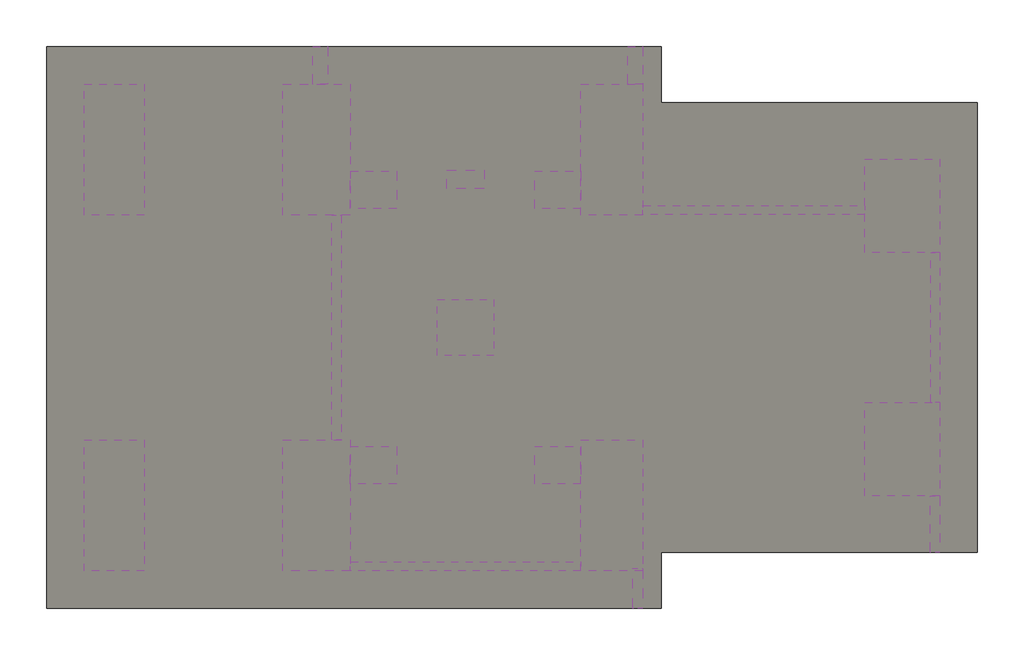
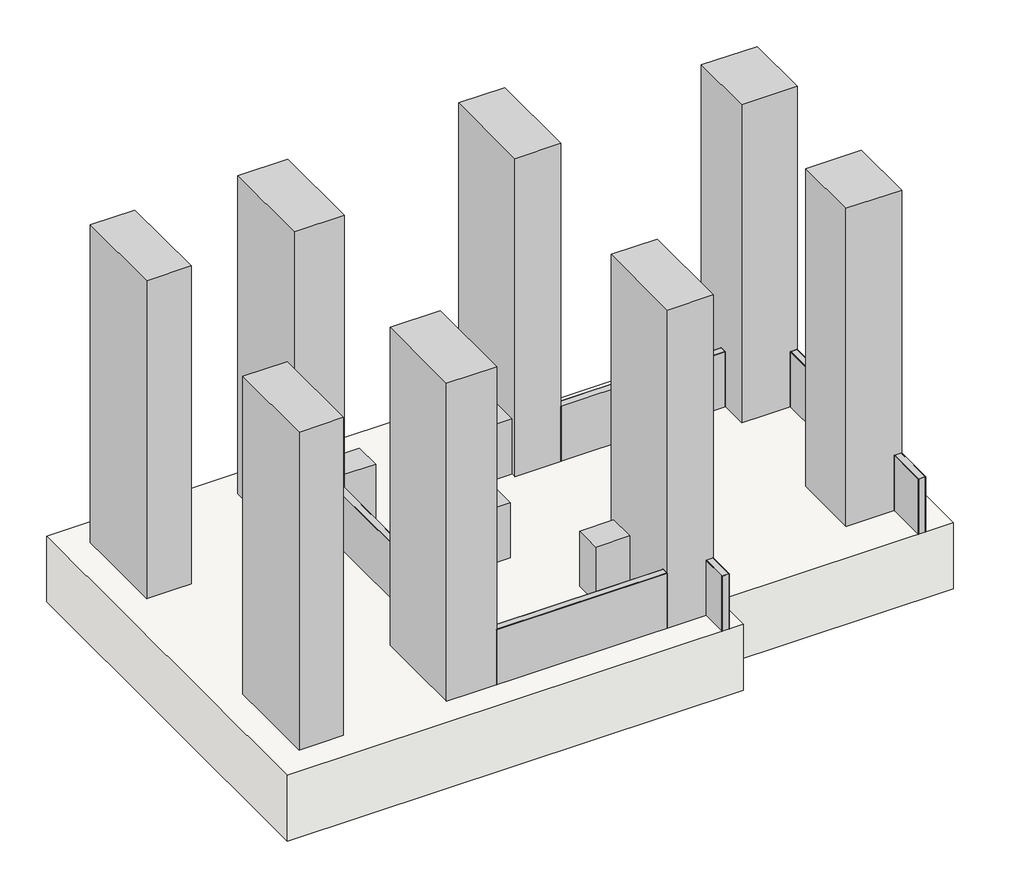
# One storey: 14 columns, 8 beams, 1 slab.
"""IFC4 building model written with IfcOpenShell, lengths in millimetres."""

import ifcopenshell
import ifcopenshell.guid

model = None  # the IFC model being written
_history = None  # IfcOwnerHistory: only IFC2X3 demands one
_inside = {}  # id of a spatial element -> (the spatial element, [elements in it])
_under = {}  # id of a project, library or spatial element -> (it, [spatial elements below it])
_declared = {}  # id of a project -> (the project, [libraries it declares])
_typed = {}  # id of a type object -> (the type object, [elements of that type])
_made_of = {}  # id of a material, layer set ... -> (it, [elements and type objects made of it])


def new_model(schema):
    """Start an empty IFC model of exactly this schema.

    Asked for "IFC4X3", IfcOpenShell would pick the latest addendum, in which some entities
    have other attributes; the version numbers below select the first issue.
    IFC2X3 requires an IfcOwnerHistory on every rooted entity: one is made here for all.
    """
    global model, _history
    if schema == "IFC4X3":
        model = ifcopenshell.file(schema_version=(4, 3, 0, 0))
    else:
        model = ifcopenshell.file(schema=schema)
    _inside.clear()
    _under.clear()
    _declared.clear()
    _typed.clear()
    _made_of.clear()
    _history = None
    if model.schema == "IFC2X3":
        org = make("IfcOrganization", Name="unknown")
        user = make(
            "IfcPersonAndOrganization",
            ThePerson=make("IfcPerson", FamilyName="unknown"),
            TheOrganization=org,
        )
        app = make(
            "IfcApplication",
            ApplicationDeveloper=org,
            Version="unknown",
            ApplicationFullName="unknown",
            ApplicationIdentifier="unknown",
        )
        _history = make(
            "IfcOwnerHistory",
            OwningUser=user,
            OwningApplication=app,
            ChangeAction="ADDED",
            CreationDate=0,
        )
    return model


def make(cls, **values):
    """One entity of the class cls with the attributes given. An attribute that is None is left unset."""
    return model.create_entity(
        cls, **{name: value for name, value in values.items() if value is not None}
    )


def rooted(cls, **values):
    """An entity with a GlobalId (a new one), such as an element, a storey or a relation."""
    return make(cls, GlobalId=ifcopenshell.guid.new(), OwnerHistory=_history, **values)


def si_unit(unit_type, name, prefix=None):
    """IfcSIUnit, for example si_unit("LENGTHUNIT", "METRE", prefix="MILLI")."""
    return make("IfcSIUnit", UnitType=unit_type, Prefix=prefix, Name=name)


def assignment(units):
    """IfcUnitAssignment: the units of a project."""
    return None if units is None else make("IfcUnitAssignment", Units=units)


def point(xyz):
    """IfcCartesianPoint."""
    return None if xyz is None else make("IfcCartesianPoint", Coordinates=xyz)


def direction(xyz):
    """IfcDirection."""
    return None if xyz is None else make("IfcDirection", DirectionRatios=xyz)


def frame(location, z_axis=None, x_axis=None):
    """IfcAxis2Placement3D, a coordinate frame: its origin and axes. An axis left out is left unset."""
    return make(
        "IfcAxis2Placement3D",
        Location=point(location),
        Axis=direction(z_axis),
        RefDirection=direction(x_axis),
    )


def origin():
    """The frame at (0, 0, 0) with its axes left unset."""
    return frame((0.0, 0.0, 0.0))


def origin_with_axes():
    """The frame at (0, 0, 0) with the z axis (0, 0, 1) and the x axis (1, 0, 0) written out."""
    return frame((0.0, 0.0, 0.0), z_axis=(0.0, 0.0, 1.0), x_axis=(1.0, 0.0, 0.0))


def place(relative_to, where):
    """IfcLocalPlacement: puts the frame where relative to a parent placement (None: the world)."""
    return make(
        "IfcLocalPlacement", PlacementRelTo=relative_to, RelativePlacement=where
    )


def context(
    kind, dimensions, precision=None, world=None, true_north=None, identifier=None
):
    """IfcGeometricRepresentationContext, for example the 3D "Model" context."""
    return make(
        "IfcGeometricRepresentationContext",
        ContextIdentifier=identifier,
        ContextType=kind,
        CoordinateSpaceDimension=dimensions,
        Precision=precision,
        WorldCoordinateSystem=world,
        TrueNorth=true_north,
    )


def project(units=None, contexts=None):
    """IfcProject with its units and contexts."""
    return rooted(
        "IfcProject",
        Name="project",
        RepresentationContexts=contexts,
        UnitsInContext=assignment(units),
    )


def spatial(cls, under=None, at=None, **own):
    """A site, building, storey or space (cls), placed at a placement, below another one or the project."""
    s = rooted(cls, ObjectPlacement=at, **own)
    if under is not None:
        _under.setdefault(under.id(), (under, []))[1].append(s)
    return s


def polyline(points):
    """IfcPolyline through the points."""
    return make("IfcPolyline", Points=[point(p) for p in points])


def outline(outer, holes=None, kind="AREA"):
    """IfcArbitraryClosedProfileDef: a profile drawn as a closed curve; with holes, ...WithVoids."""
    if holes is None:
        return make("IfcArbitraryClosedProfileDef", ProfileType=kind, OuterCurve=outer)
    return make(
        "IfcArbitraryProfileDefWithVoids",
        ProfileType=kind,
        OuterCurve=outer,
        InnerCurves=holes,
    )


def extrude(swept, where, along, depth):
    """IfcExtrudedAreaSolid: the profile swept, set in the frame where, extruded along a direction by depth."""
    return make(
        "IfcExtrudedAreaSolid",
        SweptArea=swept,
        Position=where,
        ExtrudedDirection=direction(along),
        Depth=depth,
    )


def faces_of(points, faces, orient=None, outer=None):
    """IfcFace entities. A face is a list of loops; a loop is a list of indices into points, from 0.

    orient and outer hold one flag for each loop. By default every Orientation is true, the
    first loop of a face is its IfcFaceOuterBound and the others are IfcFaceBound.
    """
    made = []
    for i, loops in enumerate(faces):
        bounds = []
        for j, loop in enumerate(loops):
            is_outer = j == 0 if outer is None else outer[i][j]
            bounds.append(
                make(
                    "IfcFaceOuterBound" if is_outer else "IfcFaceBound",
                    Bound=make("IfcPolyLoop", Polygon=[points[k] for k in loop]),
                    Orientation=True if orient is None else orient[i][j],
                )
            )
        made.append(make("IfcFace", Bounds=bounds))
    return made


def faceted_brep(points, faces, orient=None, outer=None, voids=None):
    """IfcFacetedBrep: a solid bounded by flat faces; with voids (closed shells), ...WithVoids."""
    shared = [point(p) for p in points]
    hull = make("IfcClosedShell", CfsFaces=faces_of(shared, faces, orient, outer))
    if voids is None:
        return make("IfcFacetedBrep", Outer=hull)
    return make(
        "IfcFacetedBrepWithVoids",
        Outer=hull,
        Voids=[
            make(cls, CfsFaces=faces_of(shared, fs, o, b)) for cls, fs, o, b in voids
        ],
    )


def shape(context_of_items, identifier, shape_type, items):
    """IfcShapeRepresentation: the items that make up one representation, for example the "Body"."""
    return make(
        "IfcShapeRepresentation",
        ContextOfItems=context_of_items,
        RepresentationIdentifier=identifier,
        RepresentationType=shape_type,
        Items=items,
    )


def source(mapping_origin, context_of_items, identifier, shape_type, items):
    """IfcRepresentationMap: a shape defined once, which mapped items show again and again."""
    return make(
        "IfcRepresentationMap",
        MappingOrigin=mapping_origin,
        MappedRepresentation=shape(context_of_items, identifier, shape_type, items),
    )


def transform(
    local_origin,
    x_axis=None,
    y_axis=None,
    z_axis=None,
    scale=None,
    scale2=None,
    scale3=None,
    uniform=True,
):
    """IfcCartesianTransformationOperator3D, or its non-uniform kind. x_axis, y_axis, z_axis: its Axis1, 2, 3."""
    if uniform:
        return make(
            "IfcCartesianTransformationOperator3D",
            Axis1=direction(x_axis),
            Axis2=direction(y_axis),
            LocalOrigin=point(local_origin),
            Scale=scale,
            Axis3=direction(z_axis),
        )
    return make(
        "IfcCartesianTransformationOperator3DnonUniform",
        Axis1=direction(x_axis),
        Axis2=direction(y_axis),
        LocalOrigin=point(local_origin),
        Scale=scale,
        Axis3=direction(z_axis),
        Scale2=scale2,
        Scale3=scale3,
    )


def mapped(mapping_source, mapping_target):
    """IfcMappedItem: shows the shape of a source again, moved by a transform."""
    return make(
        "IfcMappedItem", MappingSource=mapping_source, MappingTarget=mapping_target
    )


def made_of(thing, what):
    """Note that an element or type object is made of a material, layer set ...; save() writes the relation."""
    if what is not None:
        _made_of.setdefault(what.id(), (what, []))[1].append(thing)
    return thing


def element(
    cls,
    number,
    at=None,
    inside=None,
    cuts=None,
    type_object=None,
    material=None,
    context=None,
    identifier="Body",
    shape_type=None,
    held_by="IfcProductDefinitionShape",
    body=None,
    shapes=None,
    **own,
):
    """One element of the class cls, such as IfcWall. Its Tag is "e" and its number.

    at: its placement. inside: the storey or other place that contains it. cuts: it is an
    opening in that element (IfcRelVoidsElement). A single representation is given by context,
    identifier, shape_type and body (its items); several are given by shapes. held_by: the class
    of the entity that holds the representations. save() writes the other relations.
    """
    e = rooted(cls, Tag="e%d" % number, ObjectPlacement=at, **own)
    if body is not None:
        shapes = [shape(context, identifier, shape_type, body)]
    if shapes is not None:
        e.Representation = make(held_by, Representations=shapes)
    if inside is not None:
        _inside.setdefault(inside.id(), (inside, []))[1].append(e)
    if cuts is not None:
        rooted(
            "IfcRelVoidsElement", RelatingBuildingElement=cuts, RelatedOpeningElement=e
        )
    if type_object is not None:
        _typed.setdefault(type_object.id(), (type_object, []))[1].append(e)
    return made_of(e, material)


def aggregate(whole, parts):
    """IfcRelAggregates: a whole, such as a stair, and the parts it consists of."""
    return rooted("IfcRelAggregates", RelatingObject=whole, RelatedObjects=parts)


def save(model, path):
    """Write the relations noted so far, then the file.

    IfcRelAggregates (storeys below a building ...), IfcRelContainedInSpatialStructure (elements
    in a storey), IfcRelDefinesByType, IfcRelAssociatesMaterial and IfcRelDeclares: one each for
    every whole, place, type object, material and project.
    """
    for whole, parts in _under.values():
        aggregate(whole, parts)
    for where, things in _inside.values():
        rooted(
            "IfcRelContainedInSpatialStructure",
            RelatedElements=things,
            RelatingStructure=where,
        )
    for kind, things in _typed.values():
        rooted("IfcRelDefinesByType", RelatedObjects=things, RelatingType=kind)
    for what, things in _made_of.values():
        rooted("IfcRelAssociatesMaterial", RelatedObjects=things, RelatingMaterial=what)
    for by, libraries in _declared.values():
        rooted("IfcRelDeclares", RelatingContext=by, RelatedDefinitions=libraries)
    model.write(path)


def beam_97304d78(model_context):
    return source(origin(), model_context, "Body", "SweptSolid", [
        extrude(outline(polyline([(200.0, -500.0), (-200.0, -500.0), (-200.0, 500.0), (200.0, 500.0), (200.0, -500.0)])), origin_with_axes(), (0.0, 0.0, 1.0), 2100.0),
        extrude(outline(polyline([(-200.0, -485.0), (-200.0, -484.0), (200.0, -484.0), (200.0, -485.0), (-200.0, -485.0)])), origin_with_axes(), (0.0, 0.0, 1.0), 2100.0),
        extrude(outline(polyline([(-200.0, -490.0), (-200.0, -489.0), (200.0, -489.0), (200.0, -490.0), (-200.0, -490.0)])), origin_with_axes(), (0.0, 0.0, 1.0), 2100.0),
        extrude(outline(polyline([(-200.0, -495.0), (-200.0, -494.0), (200.0, -494.0), (200.0, -495.0), (-200.0, -495.0)])), origin_with_axes(), (0.0, 0.0, 1.0), 2100.0),
        extrude(outline(polyline([(-200.0, 485.0), (200.0, 485.0), (200.0, 484.0), (-200.0, 484.0), (-200.0, 485.0)])), origin_with_axes(), (0.0, 0.0, 1.0), 2100.0),
        extrude(outline(polyline([(-200.0, 490.0), (200.0, 490.0), (200.0, 489.0), (-200.0, 489.0), (-200.0, 490.0)])), origin_with_axes(), (0.0, 0.0, 1.0), 2100.0),
        extrude(outline(polyline([(-200.0, 495.0), (200.0, 495.0), (200.0, 494.0), (-200.0, 494.0), (-200.0, 495.0)])), origin_with_axes(), (0.0, 0.0, 1.0), 2100.0),
        extrude(outline(polyline([(184.0, 500.0), (185.0, 500.0), (185.0, -500.0), (184.0, -500.0), (184.0, 500.0)])), origin_with_axes(), (0.0, 0.0, 1.0), 2100.0),
        extrude(outline(polyline([(189.0, 500.0), (190.0, 500.0), (190.0, -500.0), (189.0, -500.0), (189.0, 500.0)])), origin_with_axes(), (0.0, 0.0, 1.0), 2100.0),
        extrude(outline(polyline([(194.0, 500.0), (195.0, 500.0), (195.0, -500.0), (194.0, -500.0), (194.0, 500.0)])), origin_with_axes(), (0.0, 0.0, 1.0), 2100.0),
        extrude(outline(polyline([(-184.0, 500.0), (-184.0, -500.0), (-185.0, -500.0), (-185.0, 500.0), (-184.0, 500.0)])), origin_with_axes(), (0.0, 0.0, 1.0), 2100.0),
        extrude(outline(polyline([(-189.0, 500.0), (-189.0, -500.0), (-190.0, -500.0), (-190.0, 500.0), (-189.0, 500.0)])), origin_with_axes(), (0.0, 0.0, 1.0), 2100.0),
        extrude(outline(polyline([(-194.0, 500.0), (-194.0, -500.0), (-195.0, -500.0), (-195.0, 500.0), (-194.0, 500.0)])), origin_with_axes(), (0.0, 0.0, 1.0), 2100.0),
    ])


def beam_3de7345f(model_context):
    return source(origin(), model_context, "Body", "SweptSolid", [
        extrude(outline(polyline([(130.0, -750.0), (-130.0, -750.0), (-130.0, 750.0), (130.0, 750.0), (130.0, -750.0)])), origin_with_axes(), (0.0, 0.0, 1.0), 2100.0),
        extrude(outline(polyline([(-130.0, -735.0), (-130.0, -734.0), (130.0, -734.0), (130.0, -735.0), (-130.0, -735.0)])), origin_with_axes(), (0.0, 0.0, 1.0), 2100.0),
        extrude(outline(polyline([(-130.0, -740.0), (-130.0, -739.0), (130.0, -739.0), (130.0, -740.0), (-130.0, -740.0)])), origin_with_axes(), (0.0, 0.0, 1.0), 2100.0),
        extrude(outline(polyline([(-130.0, -745.0), (-130.0, -744.0), (130.0, -744.0), (130.0, -745.0), (-130.0, -745.0)])), origin_with_axes(), (0.0, 0.0, 1.0), 2100.0),
        extrude(outline(polyline([(-130.0, 735.0), (130.0, 735.0), (130.0, 734.0), (-130.0, 734.0), (-130.0, 735.0)])), origin_with_axes(), (0.0, 0.0, 1.0), 2100.0),
        extrude(outline(polyline([(-130.0, 740.0), (130.0, 740.0), (130.0, 739.0), (-130.0, 739.0), (-130.0, 740.0)])), origin_with_axes(), (0.0, 0.0, 1.0), 2100.0),
        extrude(outline(polyline([(-130.0, 745.0), (130.0, 745.0), (130.0, 744.0), (-130.0, 744.0), (-130.0, 745.0)])), origin_with_axes(), (0.0, 0.0, 1.0), 2100.0),
        extrude(outline(polyline([(114.0, 750.0), (115.0, 750.0), (115.0, -750.0), (114.0, -750.0), (114.0, 750.0)])), origin_with_axes(), (0.0, 0.0, 1.0), 2100.0),
        extrude(outline(polyline([(119.0, 750.0), (120.0, 750.0), (120.0, -750.0), (119.0, -750.0), (119.0, 750.0)])), origin_with_axes(), (0.0, 0.0, 1.0), 2100.0),
        extrude(outline(polyline([(124.0, 750.0), (125.0, 750.0), (125.0, -750.0), (124.0, -750.0), (124.0, 750.0)])), origin_with_axes(), (0.0, 0.0, 1.0), 2100.0),
        extrude(outline(polyline([(-114.0, 750.0), (-114.0, -750.0), (-115.0, -750.0), (-115.0, 750.0), (-114.0, 750.0)])), origin_with_axes(), (0.0, 0.0, 1.0), 2100.0),
        extrude(outline(polyline([(-119.0, 750.0), (-119.0, -750.0), (-120.0, -750.0), (-120.0, 750.0), (-119.0, 750.0)])), origin_with_axes(), (0.0, 0.0, 1.0), 2100.0),
        extrude(outline(polyline([(-124.0, 750.0), (-124.0, -750.0), (-125.0, -750.0), (-125.0, 750.0), (-124.0, 750.0)])), origin_with_axes(), (0.0, 0.0, 1.0), 2100.0),
    ])


def beam_92c4ef8c(model_context):
    return source(origin(), model_context, "Body", "SweptSolid", [
        extrude(outline(polyline([(130.0, -535.0), (-130.0, -535.0), (-130.0, 535.0), (130.0, 535.0), (130.0, -535.0)])), origin_with_axes(), (0.0, 0.0, 1.0), 2100.0),
        extrude(outline(polyline([(-130.0, -520.0), (-130.0, -519.0), (130.0, -519.0), (130.0, -520.0), (-130.0, -520.0)])), origin_with_axes(), (0.0, 0.0, 1.0), 2100.0),
        extrude(outline(polyline([(-130.0, -525.0), (-130.0, -524.0), (130.0, -524.0), (130.0, -525.0), (-130.0, -525.0)])), origin_with_axes(), (0.0, 0.0, 1.0), 2100.0),
        extrude(outline(polyline([(-130.0, -530.0), (-130.0, -529.0), (130.0, -529.0), (130.0, -530.0), (-130.0, -530.0)])), origin_with_axes(), (0.0, 0.0, 1.0), 2100.0),
        extrude(outline(polyline([(-130.0, 520.0), (130.0, 520.0), (130.0, 519.0), (-130.0, 519.0), (-130.0, 520.0)])), origin_with_axes(), (0.0, 0.0, 1.0), 2100.0),
        extrude(outline(polyline([(-130.0, 525.0), (130.0, 525.0), (130.0, 524.0), (-130.0, 524.0), (-130.0, 525.0)])), origin_with_axes(), (0.0, 0.0, 1.0), 2100.0),
        extrude(outline(polyline([(-130.0, 530.0), (130.0, 530.0), (130.0, 529.0), (-130.0, 529.0), (-130.0, 530.0)])), origin_with_axes(), (0.0, 0.0, 1.0), 2100.0),
        extrude(outline(polyline([(114.0, 535.0), (115.0, 535.0), (115.0, -535.0), (114.0, -535.0), (114.0, 535.0)])), origin_with_axes(), (0.0, 0.0, 1.0), 2100.0),
        extrude(outline(polyline([(119.0, 535.0), (120.0, 535.0), (120.0, -535.0), (119.0, -535.0), (119.0, 535.0)])), origin_with_axes(), (0.0, 0.0, 1.0), 2100.0),
        extrude(outline(polyline([(124.0, 535.0), (125.0, 535.0), (125.0, -535.0), (124.0, -535.0), (124.0, 535.0)])), origin_with_axes(), (0.0, 0.0, 1.0), 2100.0),
        extrude(outline(polyline([(-114.0, 535.0), (-114.0, -535.0), (-115.0, -535.0), (-115.0, 535.0), (-114.0, 535.0)])), origin_with_axes(), (0.0, 0.0, 1.0), 2100.0),
        extrude(outline(polyline([(-119.0, 535.0), (-119.0, -535.0), (-120.0, -535.0), (-120.0, 535.0), (-119.0, 535.0)])), origin_with_axes(), (0.0, 0.0, 1.0), 2100.0),
        extrude(outline(polyline([(-124.0, 535.0), (-124.0, -535.0), (-125.0, -535.0), (-125.0, 535.0), (-124.0, 535.0)])), origin_with_axes(), (0.0, 0.0, 1.0), 2100.0),
    ])


def beam_6e677b00(model_context):
    return source(origin(), model_context, "Body", "SweptSolid", [
        extrude(outline(polyline([(125.0, -3000.0), (-125.0, -3000.0), (-125.0, 3000.0), (125.0, 3000.0), (125.0, -3000.0)])), origin_with_axes(), (0.0, 0.0, 1.0), 2100.0),
        extrude(outline(polyline([(-125.0, -2985.0), (-125.0, -2984.0), (125.0, -2984.0), (125.0, -2985.0), (-125.0, -2985.0)])), origin_with_axes(), (0.0, 0.0, 1.0), 2100.0),
        extrude(outline(polyline([(-125.0, -2990.0), (-125.0, -2989.0), (125.0, -2989.0), (125.0, -2990.0), (-125.0, -2990.0)])), origin_with_axes(), (0.0, 0.0, 1.0), 2100.0),
        extrude(outline(polyline([(-125.0, -2995.0), (-125.0, -2994.0), (125.0, -2994.0), (125.0, -2995.0), (-125.0, -2995.0)])), origin_with_axes(), (0.0, 0.0, 1.0), 2100.0),
        extrude(outline(polyline([(-125.0, 2985.0), (125.0, 2985.0), (125.0, 2984.0), (-125.0, 2984.0), (-125.0, 2985.0)])), origin_with_axes(), (0.0, 0.0, 1.0), 2100.0),
        extrude(outline(polyline([(-125.0, 2990.0), (125.0, 2990.0), (125.0, 2989.0), (-125.0, 2989.0), (-125.0, 2990.0)])), origin_with_axes(), (0.0, 0.0, 1.0), 2100.0),
        extrude(outline(polyline([(-125.0, 2995.0), (125.0, 2995.0), (125.0, 2994.0), (-125.0, 2994.0), (-125.0, 2995.0)])), origin_with_axes(), (0.0, 0.0, 1.0), 2100.0),
        extrude(outline(polyline([(109.0, 3000.0), (110.0, 3000.0), (110.0, -3000.0), (109.0, -3000.0), (109.0, 3000.0)])), origin_with_axes(), (0.0, 0.0, 1.0), 2100.0),
        extrude(outline(polyline([(114.0, 3000.0), (115.0, 3000.0), (115.0, -3000.0), (114.0, -3000.0), (114.0, 3000.0)])), origin_with_axes(), (0.0, 0.0, 1.0), 2100.0),
        extrude(outline(polyline([(119.0, 3000.0), (120.0, 3000.0), (120.0, -3000.0), (119.0, -3000.0), (119.0, 3000.0)])), origin_with_axes(), (0.0, 0.0, 1.0), 2100.0),
        extrude(outline(polyline([(-109.0, 3000.0), (-109.0, -3000.0), (-110.0, -3000.0), (-110.0, 3000.0), (-109.0, 3000.0)])), origin_with_axes(), (0.0, 0.0, 1.0), 2100.0),
        extrude(outline(polyline([(-114.0, 3000.0), (-114.0, -3000.0), (-115.0, -3000.0), (-115.0, 3000.0), (-114.0, 3000.0)])), origin_with_axes(), (0.0, 0.0, 1.0), 2100.0),
        extrude(outline(polyline([(-119.0, 3000.0), (-119.0, -3000.0), (-120.0, -3000.0), (-120.0, 3000.0), (-119.0, 3000.0)])), origin_with_axes(), (0.0, 0.0, 1.0), 2100.0),
    ])


def beam_d786ea5f(model_context):
    return source(origin(), model_context, "Body", "SweptSolid", [
        extrude(outline(polyline([(125.0, -3072.5), (-125.0, -3072.5), (-125.0, 3072.5), (125.0, 3072.5), (125.0, -3072.5)])), origin_with_axes(), (0.0, 0.0, 1.0), 2100.0),
        extrude(outline(polyline([(-125.0, -3057.5), (-125.0, -3056.5), (125.0, -3056.5), (125.0, -3057.5), (-125.0, -3057.5)])), origin_with_axes(), (0.0, 0.0, 1.0), 2100.0),
        extrude(outline(polyline([(-125.0, -3062.5), (-125.0, -3061.5), (125.0, -3061.5), (125.0, -3062.5), (-125.0, -3062.5)])), origin_with_axes(), (0.0, 0.0, 1.0), 2100.0),
        extrude(outline(polyline([(-125.0, -3067.5), (-125.0, -3066.5), (125.0, -3066.5), (125.0, -3067.5), (-125.0, -3067.5)])), origin_with_axes(), (0.0, 0.0, 1.0), 2100.0),
        extrude(outline(polyline([(-125.0, 3057.5), (125.0, 3057.5), (125.0, 3056.5), (-125.0, 3056.5), (-125.0, 3057.5)])), origin_with_axes(), (0.0, 0.0, 1.0), 2100.0),
        extrude(outline(polyline([(-125.0, 3062.5), (125.0, 3062.5), (125.0, 3061.5), (-125.0, 3061.5), (-125.0, 3062.5)])), origin_with_axes(), (0.0, 0.0, 1.0), 2100.0),
        extrude(outline(polyline([(-125.0, 3067.5), (125.0, 3067.5), (125.0, 3066.5), (-125.0, 3066.5), (-125.0, 3067.5)])), origin_with_axes(), (0.0, 0.0, 1.0), 2100.0),
        extrude(outline(polyline([(109.0, 3072.5), (110.0, 3072.5), (110.0, -3072.5), (109.0, -3072.5), (109.0, 3072.5)])), origin_with_axes(), (0.0, 0.0, 1.0), 2100.0),
        extrude(outline(polyline([(114.0, 3072.5), (115.0, 3072.5), (115.0, -3072.5), (114.0, -3072.5), (114.0, 3072.5)])), origin_with_axes(), (0.0, 0.0, 1.0), 2100.0),
        extrude(outline(polyline([(119.0, 3072.5), (120.0, 3072.5), (120.0, -3072.5), (119.0, -3072.5), (119.0, 3072.5)])), origin_with_axes(), (0.0, 0.0, 1.0), 2100.0),
        extrude(outline(polyline([(-109.0, 3072.5), (-109.0, -3072.5), (-110.0, -3072.5), (-110.0, 3072.5), (-109.0, 3072.5)])), origin_with_axes(), (0.0, 0.0, 1.0), 2100.0),
        extrude(outline(polyline([(-114.0, 3072.5), (-114.0, -3072.5), (-115.0, -3072.5), (-115.0, 3072.5), (-114.0, 3072.5)])), origin_with_axes(), (0.0, 0.0, 1.0), 2100.0),
        extrude(outline(polyline([(-119.0, 3072.5), (-119.0, -3072.5), (-120.0, -3072.5), (-120.0, 3072.5), (-119.0, 3072.5)])), origin_with_axes(), (0.0, 0.0, 1.0), 2100.0),
    ])


def beam_991fab6d(model_context):
    return source(origin(), model_context, "Body", "SweptSolid", [
        extrude(outline(polyline([(125.0, -2965.0), (-125.0, -2965.0), (-125.0, 2965.0), (125.0, 2965.0), (125.0, -2965.0)])), origin_with_axes(), (0.0, 0.0, 1.0), 2100.0),
        extrude(outline(polyline([(-125.0, -2950.0), (-125.0, -2949.0), (125.0, -2949.0), (125.0, -2950.0), (-125.0, -2950.0)])), origin_with_axes(), (0.0, 0.0, 1.0), 2100.0),
        extrude(outline(polyline([(-125.0, -2955.0), (-125.0, -2954.0), (125.0, -2954.0), (125.0, -2955.0), (-125.0, -2955.0)])), origin_with_axes(), (0.0, 0.0, 1.0), 2100.0),
        extrude(outline(polyline([(-125.0, -2960.0), (-125.0, -2959.0), (125.0, -2959.0), (125.0, -2960.0), (-125.0, -2960.0)])), origin_with_axes(), (0.0, 0.0, 1.0), 2100.0),
        extrude(outline(polyline([(-125.0, 2950.0), (125.0, 2950.0), (125.0, 2949.0), (-125.0, 2949.0), (-125.0, 2950.0)])), origin_with_axes(), (0.0, 0.0, 1.0), 2100.0),
        extrude(outline(polyline([(-125.0, 2955.0), (125.0, 2955.0), (125.0, 2954.0), (-125.0, 2954.0), (-125.0, 2955.0)])), origin_with_axes(), (0.0, 0.0, 1.0), 2100.0),
        extrude(outline(polyline([(-125.0, 2960.0), (125.0, 2960.0), (125.0, 2959.0), (-125.0, 2959.0), (-125.0, 2960.0)])), origin_with_axes(), (0.0, 0.0, 1.0), 2100.0),
        extrude(outline(polyline([(109.0, 2965.0), (110.0, 2965.0), (110.0, -2965.0), (109.0, -2965.0), (109.0, 2965.0)])), origin_with_axes(), (0.0, 0.0, 1.0), 2100.0),
        extrude(outline(polyline([(114.0, 2965.0), (115.0, 2965.0), (115.0, -2965.0), (114.0, -2965.0), (114.0, 2965.0)])), origin_with_axes(), (0.0, 0.0, 1.0), 2100.0),
        extrude(outline(polyline([(119.0, 2965.0), (120.0, 2965.0), (120.0, -2965.0), (119.0, -2965.0), (119.0, 2965.0)])), origin_with_axes(), (0.0, 0.0, 1.0), 2100.0),
        extrude(outline(polyline([(-109.0, 2965.0), (-109.0, -2965.0), (-110.0, -2965.0), (-110.0, 2965.0), (-109.0, 2965.0)])), origin_with_axes(), (0.0, 0.0, 1.0), 2100.0),
        extrude(outline(polyline([(-114.0, 2965.0), (-114.0, -2965.0), (-115.0, -2965.0), (-115.0, 2965.0), (-114.0, 2965.0)])), origin_with_axes(), (0.0, 0.0, 1.0), 2100.0),
        extrude(outline(polyline([(-119.0, 2965.0), (-119.0, -2965.0), (-120.0, -2965.0), (-120.0, 2965.0), (-119.0, 2965.0)])), origin_with_axes(), (0.0, 0.0, 1.0), 2100.0),
    ])


def beam_d64feadd(model_context):
    return source(origin(), model_context, "Body", "SweptSolid", [
        extrude(outline(polyline([(125.0, -2000.0), (-125.0, -2000.0), (-125.0, 2000.0), (125.0, 2000.0), (125.0, -2000.0)])), origin_with_axes(), (0.0, 0.0, 1.0), 2100.0),
        extrude(outline(polyline([(-125.0, -1985.0), (-125.0, -1984.0), (125.0, -1984.0), (125.0, -1985.0), (-125.0, -1985.0)])), origin_with_axes(), (0.0, 0.0, 1.0), 2100.0),
        extrude(outline(polyline([(-125.0, -1990.0), (-125.0, -1989.0), (125.0, -1989.0), (125.0, -1990.0), (-125.0, -1990.0)])), origin_with_axes(), (0.0, 0.0, 1.0), 2100.0),
        extrude(outline(polyline([(-125.0, -1995.0), (-125.0, -1994.0), (125.0, -1994.0), (125.0, -1995.0), (-125.0, -1995.0)])), origin_with_axes(), (0.0, 0.0, 1.0), 2100.0),
        extrude(outline(polyline([(-125.0, 1985.0), (125.0, 1985.0), (125.0, 1984.0), (-125.0, 1984.0), (-125.0, 1985.0)])), origin_with_axes(), (0.0, 0.0, 1.0), 2100.0),
        extrude(outline(polyline([(-125.0, 1990.0), (125.0, 1990.0), (125.0, 1989.0), (-125.0, 1989.0), (-125.0, 1990.0)])), origin_with_axes(), (0.0, 0.0, 1.0), 2100.0),
        extrude(outline(polyline([(-125.0, 1995.0), (125.0, 1995.0), (125.0, 1994.0), (-125.0, 1994.0), (-125.0, 1995.0)])), origin_with_axes(), (0.0, 0.0, 1.0), 2100.0),
        extrude(outline(polyline([(109.0, 2000.0), (110.0, 2000.0), (110.0, -2000.0), (109.0, -2000.0), (109.0, 2000.0)])), origin_with_axes(), (0.0, 0.0, 1.0), 2100.0),
        extrude(outline(polyline([(114.0, 2000.0), (115.0, 2000.0), (115.0, -2000.0), (114.0, -2000.0), (114.0, 2000.0)])), origin_with_axes(), (0.0, 0.0, 1.0), 2100.0),
        extrude(outline(polyline([(119.0, 2000.0), (120.0, 2000.0), (120.0, -2000.0), (119.0, -2000.0), (119.0, 2000.0)])), origin_with_axes(), (0.0, 0.0, 1.0), 2100.0),
        extrude(outline(polyline([(-109.0, 2000.0), (-109.0, -2000.0), (-110.0, -2000.0), (-110.0, 2000.0), (-109.0, 2000.0)])), origin_with_axes(), (0.0, 0.0, 1.0), 2100.0),
        extrude(outline(polyline([(-114.0, 2000.0), (-114.0, -2000.0), (-115.0, -2000.0), (-115.0, 2000.0), (-114.0, 2000.0)])), origin_with_axes(), (0.0, 0.0, 1.0), 2100.0),
        extrude(outline(polyline([(-119.0, 2000.0), (-119.0, -2000.0), (-120.0, -2000.0), (-120.0, 2000.0), (-119.0, 2000.0)])), origin_with_axes(), (0.0, 0.0, 1.0), 2100.0),
    ])


def concrete_rectangular_column_cl111_1000x500_pd3_b8057e20(model_context):
    return source(origin(), model_context, "Body", "SweptSolid", [
        extrude(outline(polyline([(500.0, 250.0), (500.0, -250.0), (-500.0, -250.0), (-500.0, 250.0), (500.0, 250.0)])), frame((0.0, 0.0, -2100.0), z_axis=(0.0, 0.0, 1.0), x_axis=(1.0, 0.0, 0.0)), (0.0, 0.0, 1.0), 2200.0),
    ])


def concrete_rectangular_column_cl111_1230x1000_pd1_d73c58a3(model_context):
    return source(origin(), model_context, "Body", "SweptSolid", [
        extrude(outline(polyline([(615.0, 500.0), (615.0, -500.0), (-615.0, -500.0), (-615.0, 500.0), (615.0, 500.0)])), frame((0.0, 0.0, -2100.0), z_axis=(0.0, 0.0, 1.0), x_axis=(1.0, 0.0, 0.0)), (0.0, 0.0, 1.0), 2100.0),
    ])


def concrete_rectangular_column_cl111_1500x1500_pd2_705c837b(model_context):
    return source(origin(), model_context, "Body", "SweptSolid", [
        extrude(outline(polyline([(750.0, 750.0), (750.0, -750.0), (-750.0, -750.0), (-750.0, 750.0), (750.0, 750.0)])), frame((0.0, 0.0, -2100.0), z_axis=(0.0, 0.0, 1.0), x_axis=(1.0, 0.0, 0.0)), (0.0, 0.0, 1.0), 2100.0),
    ])


def concrete_rectangular_column_cl111_1600x3500_c1_e9203d13(model_context):
    return source(origin(), model_context, "Body", "SweptSolid", [
        extrude(outline(polyline([(800.0, 1750.0), (800.0, -1750.0), (-800.0, -1750.0), (-800.0, 1750.0), (800.0, 1750.0)])), frame((0.0, 0.0, -2100.0), z_axis=(0.0, 0.0, 1.0), x_axis=(1.0, 0.0, 0.0)), (0.0, 0.0, 1.0), 12100.0),
    ])


def concrete_rectangular_column_cl111_1800x3500_c2_0d95458a(model_context):
    return source(origin(), model_context, "Body", "SweptSolid", [
        extrude(outline(polyline([(900.0, 1750.0), (900.0, -1750.0), (-900.0, -1750.0), (-900.0, 1750.0), (900.0, 1750.0)])), frame((0.0, 0.0, -2100.0), z_axis=(0.0, 0.0, 1.0), x_axis=(1.0, 0.0, 0.0)), (0.0, 0.0, 1.0), 12100.0),
    ])


model = new_model("IFC4")

# Units and contexts
model_context = context("Model", 3, world=origin())
ifc_project = project(units=[si_unit("LENGTHUNIT", "METRE", prefix="MILLI")], contexts=[model_context])

# Site, building, storey
site = spatial("IfcSite", under=ifc_project)
building = spatial("IfcBuilding", under=site)
storey = spatial("IfcBuildingStorey", under=building, Name="B.O.FDN.", Elevation=-4600.0)

# Beams
placement = place(None, origin())
beam_shape = beam_97304d78(model_context)
element("IfcBeam", 1, ObjectType="LF02ZBK001_DIKE WALL_RC : Dike_Thk.400_EW2", at=placement, inside=storey, context=model_context, shape_type="MappedRepresentation", body=[
    mapped(beam_shape, transform((8700.0, 18999.5208589, -2100.0), x_axis=(1.0, 0.0, 0.0), y_axis=(0.0, 1.0, 0.0), z_axis=(0.0, 0.0, 1.0))),
])
element("IfcBeam", 2, ObjectType="LF02ZBK001_DIKE WALL_RC : Dike_Thk.400_EW2", at=placement, inside=storey, context=model_context, shape_type="MappedRepresentation", body=[
    mapped(beam_shape, transform((17100.0, 18999.5208589, -2100.0), x_axis=(1.0, 0.0, 0.0), y_axis=(0.0, 1.0, 0.0), z_axis=(0.0, 0.0, 1.0))),
])
beam_2_shape = beam_3de7345f(model_context)
element("IfcBeam", 3, ObjectType="LF02ZBK001_DIKE WALL_RC : Dike_Thk.260_EW1", at=placement, inside=storey, context=model_context, shape_type="MappedRepresentation", body=[
    mapped(beam_2_shape, transform((25100.0, 6749.5208589, -2100.0), x_axis=(1.0, 0.0, 0.0), y_axis=(0.0, 1.0, 0.0), z_axis=(0.0, 0.0, 1.0))),
])
beam_3_shape = beam_92c4ef8c(model_context)
element("IfcBeam", 4, ObjectType="LF02ZBK001_DIKE WALL_RC : Dike_Thk.260_EW1", at=placement, inside=storey, context=model_context, shape_type="MappedRepresentation", body=[
    mapped(beam_3_shape, transform((17170.0, 5034.5208589, -2100.0), x_axis=(1.0, 0.0, 0.0), y_axis=(0.0, 1.0, 0.0), z_axis=(0.0, 0.0, 1.0))),
])
beam_4_shape = beam_6e677b00(model_context)
element("IfcBeam", 5, ObjectType="LF02ZBK001_DIKE WALL_RC : Dike_Thk.250_EW3", at=placement, inside=storey, context=model_context, shape_type="MappedRepresentation", body=[
    mapped(beam_4_shape, transform((9130.0, 11999.5208589, -2100.0), x_axis=(1.0, 0.0, 0.0), y_axis=(0.0, 1.0, 0.0), z_axis=(0.0, 0.0, 1.0))),
])
beam_5_shape = beam_d786ea5f(model_context)
element("IfcBeam", 6, ObjectType="LF02ZBK001_DIKE WALL_RC : Dike_Thk.250_EW3", at=placement, inside=storey, context=model_context, shape_type="MappedRepresentation", body=[
    mapped(beam_5_shape, transform((12577.5, 5624.5208589, -2100.0), x_axis=(0.0, 1.0, 0.0), y_axis=(-1.0, 0.0, 0.0), z_axis=(0.0, 0.0, 1.0))),
])
beam_6_shape = beam_991fab6d(model_context)
element("IfcBeam", 7, ObjectType="LF02ZBK001_DIKE WALL_RC : Dike_Thk.250_EW3", at=placement, inside=storey, context=model_context, shape_type="MappedRepresentation", body=[
    mapped(beam_6_shape, transform((20265.0, 15132.4579995, -2100.0), x_axis=(0.0, -1.0, 0.0), y_axis=(1.0, 0.0, 0.0), z_axis=(0.0, 0.0, 1.0))),
])
beam_7_shape = beam_d64feadd(model_context)
element("IfcBeam", 8, ObjectType="LF02ZBK001_DIKE WALL_RC : Dike_Thk.250_EW3", at=placement, inside=storey, context=model_context, shape_type="MappedRepresentation", body=[
    mapped(beam_7_shape, transform((25105.0, 11999.5208589, -2100.0), x_axis=(1.0, 0.0, 0.0), y_axis=(0.0, 1.0, 0.0), z_axis=(0.0, 0.0, 1.0))),
])

# Columns
concrete_rectangular_column_cl111_1000x500_pd3_shape = concrete_rectangular_column_cl111_1000x500_pd3_b8057e20(model_context)
element("IfcColumn", 9, ObjectType="Concrete-Rectangular-Column : CL111_1000x500_PD3", at=placement, inside=storey, context=model_context, shape_type="MappedRepresentation", body=[
    mapped(concrete_rectangular_column_cl111_1000x500_pd3_shape, transform((12577.5, 15956.5208589, 0.0), x_axis=(1.0, 0.0, 0.0), y_axis=(0.0, 1.0, 0.0), z_axis=(0.0, 0.0, 1.0))),
])
concrete_rectangular_column_cl111_1230x1000_pd1_shape = concrete_rectangular_column_cl111_1230x1000_pd1_d73c58a3(model_context)
element("IfcColumn", 10, ObjectType="Concrete-Rectangular-Column : CL111_1230x1000_PD1", at=placement, inside=storey, context=model_context, shape_type="MappedRepresentation", body=[
    mapped(concrete_rectangular_column_cl111_1230x1000_pd1_shape, transform((10120.0, 15667.5208589, 0.0), x_axis=(1.0, 0.0, 0.0), y_axis=(0.0, 1.0, 0.0), z_axis=(0.0, 0.0, 1.0))),
])
element("IfcColumn", 11, ObjectType="Concrete-Rectangular-Column : CL111_1230x1000_PD1", at=placement, inside=storey, context=model_context, shape_type="MappedRepresentation", body=[
    mapped(concrete_rectangular_column_cl111_1230x1000_pd1_shape, transform((15035.0, 15667.5208589, 0.0), x_axis=(1.0, 0.0, 0.0), y_axis=(0.0, 1.0, 0.0), z_axis=(0.0, 0.0, 1.0))),
])
element("IfcColumn", 12, ObjectType="Concrete-Rectangular-Column : CL111_1230x1000_PD1", at=placement, inside=storey, context=model_context, shape_type="MappedRepresentation", body=[
    mapped(concrete_rectangular_column_cl111_1230x1000_pd1_shape, transform((10120.0, 8331.5208589, 0.0), x_axis=(1.0, 0.0, 0.0), y_axis=(0.0, 1.0, 0.0), z_axis=(0.0, 0.0, 1.0))),
])
element("IfcColumn", 13, ObjectType="Concrete-Rectangular-Column : CL111_1230x1000_PD1", at=placement, inside=storey, context=model_context, shape_type="MappedRepresentation", body=[
    mapped(concrete_rectangular_column_cl111_1230x1000_pd1_shape, transform((15035.0, 8331.5208589, 0.0), x_axis=(1.0, 0.0, 0.0), y_axis=(0.0, 1.0, 0.0), z_axis=(0.0, 0.0, 1.0))),
])
concrete_rectangular_column_cl111_1500x1500_pd2_shape = concrete_rectangular_column_cl111_1500x1500_pd2_705c837b(model_context)
element("IfcColumn", 14, ObjectType="Concrete-Rectangular-Column : CL111_1500x1500_PD2", at=placement, inside=storey, context=model_context, shape_type="MappedRepresentation", body=[
    mapped(concrete_rectangular_column_cl111_1500x1500_pd2_shape, transform((12577.5, 11999.5208589, 0.0), x_axis=(1.0, 0.0, 0.0), y_axis=(0.0, 1.0, 0.0), z_axis=(0.0, 0.0, 1.0))),
])
concrete_rectangular_column_cl111_1600x3500_c1_shape = concrete_rectangular_column_cl111_1600x3500_c1_e9203d13(model_context)
element("IfcColumn", 15, ObjectType="Concrete-Rectangular-Column : CL111_1600x3500_C1", at=placement, inside=storey, context=model_context, shape_type="MappedRepresentation", body=[
    mapped(concrete_rectangular_column_cl111_1600x3500_c1_shape, transform((3200.0, 16749.5208589, 0.0), x_axis=(1.0, 0.0, 0.0), y_axis=(0.0, 1.0, 0.0), z_axis=(0.0, 0.0, 1.0))),
])
element("IfcColumn", 16, ObjectType="Concrete-Rectangular-Column : CL111_1600x3500_C1", at=placement, inside=storey, context=model_context, shape_type="MappedRepresentation", body=[
    mapped(concrete_rectangular_column_cl111_1600x3500_c1_shape, transform((3200.0, 7249.5208589, 0.0), x_axis=(1.0, 0.0, 0.0), y_axis=(0.0, 1.0, 0.0), z_axis=(0.0, 0.0, 1.0))),
])
element("IfcColumn", 17, ObjectType="Concrete-Rectangular-Column : CL111_1650x3500_C3", at=placement, inside=storey, context=model_context, shape_type="SweptSolid", body=[
    extrude(outline(polyline([(17300.0, 18499.5208589), (17300.0, 14999.5208589), (15650.0, 14999.5208589), (15650.0, 18499.5208589), (17300.0, 18499.5208589)])), frame((0.0, 0.0, -2100.0), z_axis=(0.0, 0.0, 1.0), x_axis=(1.0, 0.0, 0.0)), (0.0, 0.0, 1.0), 12100.0),
])
element("IfcColumn", 18, ObjectType="Concrete-Rectangular-Column : CL111_1650x3500_C3", at=placement, inside=storey, context=model_context, shape_type="SweptSolid", body=[
    extrude(outline(polyline([(17300.0, 8999.5208589), (17300.0, 5499.5208589), (15650.0, 5499.5208589), (15650.0, 8999.5208589), (17300.0, 8999.5208589)])), frame((0.0, 0.0, -2100.0), z_axis=(0.0, 0.0, 1.0), x_axis=(1.0, 0.0, 0.0)), (0.0, 0.0, 1.0), 12100.0),
])
concrete_rectangular_column_cl111_1800x3500_c2_shape = concrete_rectangular_column_cl111_1800x3500_c2_0d95458a(model_context)
element("IfcColumn", 19, ObjectType="Concrete-Rectangular-Column : CL111_1800x3500_C2", at=placement, inside=storey, context=model_context, shape_type="MappedRepresentation", body=[
    mapped(concrete_rectangular_column_cl111_1800x3500_c2_shape, transform((8605.0, 16749.5208589, 0.0), x_axis=(1.0, 0.0, 0.0), y_axis=(0.0, 1.0, 0.0), z_axis=(0.0, 0.0, 1.0))),
])
element("IfcColumn", 20, ObjectType="Concrete-Rectangular-Column : CL111_1800x3500_C2", at=placement, inside=storey, context=model_context, shape_type="MappedRepresentation", body=[
    mapped(concrete_rectangular_column_cl111_1800x3500_c2_shape, transform((8605.0, 7249.5208589, 0.0), x_axis=(1.0, 0.0, 0.0), y_axis=(0.0, 1.0, 0.0), z_axis=(0.0, 0.0, 1.0))),
])
element("IfcColumn", 21, ObjectType="Concrete-Rectangular-Column : CL111_2000x2500_C4", at=placement, inside=storey, context=model_context, shape_type="Brep", body=[
    faceted_brep([(25230.0, 16499.5208589, -2100.0), (25230.0, 13999.5208589, -2100.0), (23230.0, 13999.5208589, -2100.0), (23230.0, 16499.5208589, -2100.0), (25230.0, 16499.5208589, 10000.0), (25230.0, 13999.5208589, 10000.0), (25230.0, 13999.5208589, 7000.0), (25230.0, 13999.5208589, 6000.0), (23230.0, 13999.5208589, 10000.0), (23230.0, 16499.5208589, 10000.0)], [[[0, 1, 2, 3]], [[4, 5, 6, 7, 1, 0]], [[5, 8, 2, 1, 7, 6]], [[8, 9, 3, 2]], [[9, 4, 0, 3]], [[4, 9, 8, 5]]]),
])
element("IfcColumn", 22, ObjectType="Concrete-Rectangular-Column : CL111_2000x2500_C4", at=placement, inside=storey, context=model_context, shape_type="SweptSolid", body=[
    extrude(outline(polyline([(25230.0, 9999.5208589), (25230.0, 7499.5208589), (23230.0, 7499.5208589), (23230.0, 9999.5208589), (25230.0, 9999.5208589)])), frame((0.0, 0.0, -2100.0), z_axis=(0.0, 0.0, 1.0), x_axis=(1.0, 0.0, 0.0)), (0.0, 0.0, 1.0), 12100.0),
])

# Slab
element("IfcSlab", 23, ObjectType="MF00_2500", at=placement, inside=storey, context=model_context, shape_type="SweptSolid", body=[
    extrude(outline(polyline([(1400.0, 4499.5208589), (1400.0, 19499.5208589), (17800.0, 19499.5208589), (17800.0, 17999.5208589), (26230.0, 17999.5208589), (26230.0, 5999.5208589), (17800.0, 5999.5208589), (17800.0, 4499.5208589), (1400.0, 4499.5208589)])), frame((0.0, 0.0, -4600.0), z_axis=(0.0, 0.0, 1.0), x_axis=(1.0, 0.0, 0.0)), (0.0, 0.0, 1.0), 2500.0),
])

save(model, "model.ifc")

# Revit data of these elements
# Project information
#   Building Name = "MAIN GATE SECURITY BUILDING"
#   Project Status = "Project Status"
#   Client Name = "현대엔지니어링"
#   Project Address = "서울시 종로구 율곡로 75(계동)"
#   Project Name = "Therma Visayas Energy Project"
#   Project Number = "-"
# Grids (mm)
#   "D": line (-3860.098, 8999.521) -> (29146.237, 8999.521)
#   "E": line (-3860.098, 2999.521) -> (29146.237, 2999.521)
#   "2": line (0, 23562.27) -> (0, 31.002)
#   "3": line (8500, 23562.27) -> (8500, 31.002)
#   "5": line (27000, 23562.27) -> (27000, 31.002)
#   "C": line (-3860.098, 15499.521) -> (29146.237, 15499.521)
#   "B": line (-3860.098, 20999.521) -> (29146.237, 20999.521)
#   "4": line (17700, 23562.27) -> (17700, 31.002)
# Type "LF02ZBK001_DIKE WALL_RC : Dike_Thk.400_EW2"
#   Dike_thk = 400 mm
#   Dike_Length [instance default] = 3000 mm
#   Dike_Hight = 2100 mm
#   c2_visible = yes
#   c3_material [instance default] = none
#   c2_material 3 [instance default] = none
#   c2_material 2 [instance default] = none
#   c2_material 1 [instance default] = none
#   c1_material [instance default] = none
#   Default Elevation = 0
# Type "LF02ZBK001_DIKE WALL_RC : Dike_Thk.260_EW1"
#   Dike_thk = 260 mm
#   Dike_Length [instance default] = 3000 mm
#   Dike_Hight = 2100 mm
#   c2_visible = yes
#   c3_material [instance default] = none
#   c2_material 3 [instance default] = none
#   c2_material 2 [instance default] = none
#   c2_material 1 [instance default] = none
#   c1_material [instance default] = none
#   Default Elevation = 0
# Type "LF02ZBK001_DIKE WALL_RC : Dike_Thk.250_EW3"
#   Dike_thk = 250 mm
#   Dike_Length [instance default] = 3000 mm
#   Dike_Hight = 2100 mm
#   c2_visible = yes
#   c3_material [instance default] = none
#   c2_material 3 [instance default] = none
#   c2_material 2 [instance default] = none
#   c2_material 1 [instance default] = none
#   c1_material [instance default] = none
#   Default Elevation = 0
# Type "Concrete-Rectangular-Column : CL111_1000x500_PD3"
#   Description = "UG 철골 기둥용 Pedestal"
#   b = 1000 mm
#   h = 500 mm
#   Width = 1000 mm
#   Length = 500 mm
#   hec_material3 [instance default] = none
#   hec_material2 [instance default] = A03AE056-00001_Bitumen/Bituminous/Asphalt Coating
#   hec_material1 [instance default] = A03AC035-00001_Form Work (3 times in use)_Flat
#   Structural Material [instance default] = A03AC032-00007_Structural Concrete_Type1_25MPa-30Mpa
# Type "Concrete-Rectangular-Column : CL111_1230x1000_PD1"
#   Description = "UG 철골 기둥용 Pedestal"
#   b = 1230 mm
#   h = 1000 mm
#   Width = 1230 mm
#   Length = 1000 mm
#   hec_material3 [instance default] = none
#   hec_material2 [instance default] = A03AE056-00001_Bitumen/Bituminous/Asphalt Coating
#   hec_material1 [instance default] = A03AC035-00001_Form Work (3 times in use)_Flat
#   Structural Material [instance default] = A03AC032-00007_Structural Concrete_Type1_25MPa-30Mpa
# Type "Concrete-Rectangular-Column : CL111_1500x1500_PD2"
#   Description = "UG 철골 기둥용 Pedestal"
#   b = 1500 mm
#   h = 1500 mm
#   Width = 1500 mm
#   Length = 1500 mm
#   hec_material3 [instance default] = none
#   hec_material2 [instance default] = A03AE056-00001_Bitumen/Bituminous/Asphalt Coating
#   hec_material1 [instance default] = A03AC035-00001_Form Work (3 times in use)_Flat
#   Structural Material [instance default] = A03AC032-00007_Structural Concrete_Type1_25MPa-30Mpa
# Type "Concrete-Rectangular-Column : CL111_1600x3500_C1"
#   Description = "UG 철골 기둥용 Pedestal"
#   b = 1600 mm
#   h = 3500 mm
#   Width = 1600 mm
#   Length = 3500 mm
#   hec_material3 [instance default] = none
#   hec_material2 [instance default] = A03AE056-00001_Bitumen/Bituminous/Asphalt Coating
#   hec_material1 [instance default] = A03AC035-00001_Form Work (3 times in use)_Flat
#   Structural Material [instance default] = A03AC032-00007_Structural Concrete_Type1_25MPa-30Mpa
# Type "Concrete-Rectangular-Column : CL111_1650x3500_C3"
#   Description = "UG 철골 기둥용 Pedestal"
#   b = 1650 mm
#   h = 3500 mm
#   Width = 1650 mm
#   Length = 3500 mm
#   hec_material3 [instance default] = none
#   hec_material2 [instance default] = A03AE056-00001_Bitumen/Bituminous/Asphalt Coating
#   hec_material1 [instance default] = A03AC035-00001_Form Work (3 times in use)_Flat
#   Structural Material [instance default] = A03AC032-00007_Structural Concrete_Type1_25MPa-30Mpa
# Type "Concrete-Rectangular-Column : CL111_1800x3500_C2"
#   Description = "UG 철골 기둥용 Pedestal"
#   b = 1800 mm
#   h = 3500 mm
#   Width = 1800 mm
#   Length = 3500 mm
#   hec_material3 [instance default] = none
#   hec_material2 [instance default] = A03AE056-00001_Bitumen/Bituminous/Asphalt Coating
#   hec_material1 [instance default] = A03AC035-00001_Form Work (3 times in use)_Flat
#   Structural Material [instance default] = A03AC032-00007_Structural Concrete_Type1_25MPa-30Mpa
# Type "Concrete-Rectangular-Column : CL111_2000x2500_C4"
#   Description = "UG 철골 기둥용 Pedestal"
#   b = 2000 mm
#   h = 2500 mm
#   Width = 2000 mm
#   Length = 2500 mm
#   hec_material3 [instance default] = none
#   hec_material2 [instance default] = A03AE056-00001_Bitumen/Bituminous/Asphalt Coating
#   hec_material1 [instance default] = A03AC035-00001_Form Work (3 times in use)_Flat
#   Structural Material [instance default] = A03AC032-00007_Structural Concrete_Type1_25MPa-30Mpa
# Type "MF00_2500"
#   Type Comments = "구조_콘크리트"
#   Layers, outside or top first: 2500 mm "14200-030101_Concrete Pouring" (function 1)
# Elements 1, 2 (IfcBeam, "LF02ZBK001_DIKE WALL_RC : Dike_Thk.400_EW2")
#   Dike_Length = 1000 mm
#   Structural Material = 콘크리트 - 현장타설 콘크리트
#   c3_material = none
#   c2_material 3 = none
#   c2_material 2 = none
#   c2_material 1 = none
#   c1_material = none
#   Phase Created = New Construction
# Element 3 (IfcBeam, "LF02ZBK001_DIKE WALL_RC : Dike_Thk.260_EW1")
#   Dike_Length = 1500 mm
#   c3_material = none
#   c2_material 3 = none
#   c2_material 2 = none
#   c2_material 1 = none
#   c1_material = none
#   Phase Created = New Construction
# Element 4 (IfcBeam, "LF02ZBK001_DIKE WALL_RC : Dike_Thk.260_EW1")
#   Dike_Length = 1070 mm
#   c3_material = none
#   c2_material 3 = none
#   c2_material 2 = none
#   c2_material 1 = none
#   c1_material = none
#   Phase Created = New Construction
# Element 5 (IfcBeam, "LF02ZBK001_DIKE WALL_RC : Dike_Thk.250_EW3")
#   Dike_Length = 6000 mm
#   c3_material = none
#   c2_material 3 = none
#   c2_material 2 = none
#   c2_material 1 = none
#   c1_material = none
#   Phase Created = New Construction
# Element 6 (IfcBeam, "LF02ZBK001_DIKE WALL_RC : Dike_Thk.250_EW3")
#   Dike_Length = 6145 mm
#   c3_material = none
#   c2_material 3 = none
#   c2_material 2 = none
#   c2_material 1 = none
#   c1_material = none
#   Phase Created = New Construction
# Element 7 (IfcBeam, "LF02ZBK001_DIKE WALL_RC : Dike_Thk.250_EW3")
#   Dike_Length = 5930 mm
#   c3_material = none
#   c2_material 3 = none
#   c2_material 2 = none
#   c2_material 1 = none
#   c1_material = none
#   Phase Created = New Construction
# Element 8 (IfcBeam, "LF02ZBK001_DIKE WALL_RC : Dike_Thk.250_EW3")
#   Dike_Length = 4000 mm
#   c3_material = none
#   c2_material 3 = none
#   c2_material 2 = none
#   c2_material 1 = none
#   c1_material = none
#   Phase Created = New Construction
# Element 9 (IfcColumn, "Concrete-Rectangular-Column : CL111_1000x500_PD3")
#   Comments = ""
#   Structural Material = 콘크리트 - 현장타설 콘크리트
#   hec_material3 = none
#   hec_material2 = none
#   hec_material1 = none
#   Phase Created = New Construction
#   Materials on its faces: "콘크리트 - 현장타설 콘크리트"
# Elements 10, 11, 12, 13 (IfcColumn, "Concrete-Rectangular-Column : CL111_1230x1000_PD1")
#   Comments = ""
#   Structural Material = 콘크리트 - 현장타설 콘크리트
#   hec_material3 = none
#   hec_material2 = none
#   hec_material1 = none
#   Phase Created = New Construction
#   Materials on its faces: "콘크리트 - 현장타설 콘크리트"
# Element 14 (IfcColumn, "Concrete-Rectangular-Column : CL111_1500x1500_PD2")
#   Comments = ""
#   Structural Material = 콘크리트 - 현장타설 콘크리트
#   hec_material3 = none
#   hec_material2 = none
#   hec_material1 = none
#   Phase Created = New Construction
#   Materials on its faces: "콘크리트 - 현장타설 콘크리트"
# Elements 15, 16 (IfcColumn, "Concrete-Rectangular-Column : CL111_1600x3500_C1")
#   Comments = ""
#   Structural Material = 콘크리트 - 현장타설 콘크리트
#   hec_material3 = none
#   hec_material2 = none
#   hec_material1 = none
#   Phase Created = New Construction
#   Materials on its faces: "콘크리트 - 현장타설 콘크리트"
# Elements 17, 18 (IfcColumn, "Concrete-Rectangular-Column : CL111_1650x3500_C3")
#   Comments = ""
#   Structural Material = 콘크리트 - 현장타설 콘크리트
#   hec_material3 = none
#   hec_material2 = none
#   hec_material1 = none
#   Phase Created = New Construction
#   Materials on its faces: "콘크리트 - 현장타설 콘크리트"
# Elements 19, 20 (IfcColumn, "Concrete-Rectangular-Column : CL111_1800x3500_C2")
#   Comments = ""
#   Structural Material = 콘크리트 - 현장타설 콘크리트
#   hec_material3 = none
#   hec_material2 = none
#   hec_material1 = none
#   Phase Created = New Construction
#   Materials on its faces: "콘크리트 - 현장타설 콘크리트"
# Elements 21, 22 (IfcColumn, "Concrete-Rectangular-Column : CL111_2000x2500_C4")
#   Comments = ""
#   Structural Material = 콘크리트 - 현장타설 콘크리트
#   hec_material3 = none
#   hec_material2 = none
#   hec_material1 = none
#   Phase Created = New Construction
#   Materials on its faces: "콘크리트 - 현장타설 콘크리트"
# Element 23 (IfcSlab, "MF00_2500")
#   Comments = ""
#   Height Offset From Level = 0 mm
#   built-in parameter 1001954 = 1
#   Phase Created = New Construction
#   Materials on its faces: "14200-030101_Concrete Pouring"
# Materials
#   "A03AE056-00001_Bitumen/Bituminous/Asphalt Coating": class "Generic", colour RGB 17 17 17, transparency 0, Description = "Damp-proofing", W00) Work Master Code = "A03AE056-00001", W01) Work Master_Lv1 = "Concrete Work", W02) Work Master_Lv2 = "Concrete Protective Coating (U/G)", W03) Work Master_Spec.1 = "Bitumen/Bituminous/Asphalt Coating", Cost = 0
#   "A03AC035-00001_Form Work (3 times in use)_Flat": class "Wood", colour RGB 149 120 74, transparency 0, Description = "Plywood", W00) Work Master Code = "A03AC035-00001", W01) Work Master_Lv1 = "Concrete Work", W02) Work Master_Lv2 = "Substructure Work", W03) Work Master_Spec.1 = "Form Work (3 times in use)", W04) Work Master_Spec.2 = "Flat Form", W05) Work Master_Spec.3 = "Dressed Lumber, Plywood or Steel Form(Wood Planks are not Allowed) incl. Chamfer", Cost = 0
#   "A03AC032-00007_Structural Concrete_Type1_25MPa-30Mpa": class "Concrete", colour RGB 176 176 176, transparency 0, Keynote = "09910.A1", Description = "Reinf. Conc.", W00) Work Master Code = "A03AC032-00007", W01) Work Master_Lv1 = "Concrete Work", W02) Work Master_Lv2 = "Substructure Work", W03) Work Master_Spec.1 = "Structural Concrete", W04) Work Master_Spec.2 = "Cement Type-1", W05) Work Master_Spec.3 = "25MPa < F'c (Cylinder Strength) ≤ 30MPa", Cost = 0
#   "14200-030101_Concrete Pouring": class "Concrete", colour RGB 176 176 176, transparency 0, Description = "Reinf. Conc.", W00) Work Master Code = "14200-030101", W01) Work Master_Lv1 = "Concrete Work", W02) Work Master_Lv2 = "Building/Shelter Foundation Work", W03) Work Master_Spec.1 = "Concrete Pouring", W04) Work Master_Spec.2 = "F'c (Cylinder Strength) > 35MPa", W05) Work Master_Spec.3 = "Cement Type-1", Cost = 0
#   "콘크리트 - 현장타설 콘크리트": class "콘크리트", colour RGB 192 192 192, transparency 0
# Room, not placed, phase "New Construction", upper offset 0 mm, lower offset 0 mm
#   Comments = ""
#   Number = "11"
#   Name = ""
#   S01) Room Name = ""
#   S02) Room Number(Project) = ""
# Room at (1577.906, 21721.343) mm, phase "New Construction", upper level "G.L", upper offset 2700 mm, lower offset 0 mm
#   Comments = ""
#   Base Finish = "RUBBER BASE(H=100)"
#   Ceiling Finish = "SUSPENDED MINERAL FIBERBOARD PANEL(GRID 600x600)"
#   Wall Finish = "LATEX PAINT ON THK.15 CEMENT PLASTER + MASONRY WALL"
#   Floor Finish = "PVC TILE W/ADHESIVE ON STEEL TROWELED CONC. SLAB"
#   Number = "UYF01R0003"
#   Name = "LOCKER ROOM"
#   F01) Building Name = "MAIN GATE SECURITY BUILDING"
#   S01) Room Name = "LOCKER ROOM"
#   S02) Room Number(Project) = "UYF01R0003"
#   S03) Floor = "GF"
#   S04) Level = "FL+0"
#   S11) Space by Function_Lv1 = "Space for Architecture"
#   S12) Space by Function_Lv2 = "Private Residential Spaces"
#   S13) Space by Function_Lv3 = "Locker Room"
#   S21) Space by Form = "Enclosed"
# Room, not placed, phase "New Construction", upper offset 0 mm, lower offset 0 mm
#   Comments = ""
#   Number = "13"
#   Name = ""
#   S01) Room Name = ""
#   S02) Room Number(Project) = ""
# Room, not placed, phase "New Construction", upper offset 0 mm, lower offset 0 mm
#   Comments = ""
#   Number = "14"
#   Name = ""
#   S01) Room Name = ""
#   S02) Room Number(Project) = ""
# Room, not placed, phase "New Construction", upper offset 0 mm, lower offset 0 mm
#   Comments = ""
#   Number = "15"
#   Name = ""
#   S01) Room Name = ""
#   S02) Room Number(Project) = ""
# Room, not placed, phase "New Construction", upper offset 0 mm, lower offset 0 mm
#   Comments = ""
#   Number = "16"
#   Name = ""
#   S01) Room Name = ""
#   S02) Room Number(Project) = ""
# Room, not placed, phase "New Construction", upper offset 0 mm, lower offset 0 mm
#   Comments = ""
#   Number = "17"
#   Name = ""
#   S01) Room Name = ""
#   S02) Room Number(Project) = ""
# Room, not placed, phase "New Construction", upper offset 0 mm, lower offset 0 mm
#   Comments = ""
#   Number = "18"
#   Name = ""
#   S01) Room Name = ""
#   S02) Room Number(Project) = ""
# Room, not placed, phase "New Construction", upper offset 0 mm, lower offset 0 mm
#   Comments = ""
#   Number = "20"
#   Name = ""
#   S01) Room Name = ""
#   S02) Room Number(Project) = ""
# Room, not placed, phase "New Construction", upper offset 0 mm, lower offset 0 mm
#   Comments = ""
#   Number = "21"
#   Name = ""
#   S01) Room Name = ""
#   S02) Room Number(Project) = ""
# Room at (5500, 19570.521) mm, phase "New Construction", upper level "G.L", upper offset 2700 mm, lower offset 0 mm
#   Comments = ""
#   Base Finish = "RUBBER BASE(H=100)"
#   Ceiling Finish = "SUSPENDED MINERAL FIBERBOARD PANEL(GRID 600x600)"
#   Wall Finish = "LATEX PAINT ON THK.15 CEMENT PLASTER + MASONRY WALL"
#   Floor Finish = "PVC TILE W/ADHESIVE ON STEEL TROWELED CONC. SLAB"
#   Number = "UYF01R0004"
#   Name = "BREAK ROOM"
#   F01) Building Name = "MAIN GATE SECURITY BUILDING"
#   S01) Room Name = "BREAK ROOM"
#   S02) Room Number(Project) = "UYF01R0004"
#   S03) Floor = "GF"
#   S04) Level = "FL+0"
#   S11) Space by Function_Lv1 = "Space for Architecture"
#   S12) Space by Function_Lv2 = "Service Activity Spaces"
#   S13) Space by Function_Lv3 = "Break Room"
#   S21) Space by Form = "Enclosed"
# Room at (8721.053, 19570.521) mm, phase "New Construction", upper level "G.L", upper offset 2700 mm, lower offset 0 mm
#   Comments = ""
#   Base Finish = "UNGLAZED CERAMIC TILE(H=100)"
#   Ceiling Finish = "SUSPENDED MOISTURE RESISTANT PANEL"
#   Wall Finish = "H=2.0m GLAZED CERAMIC TILE ON THK.15 CEMENT PLASTER"
#   Floor Finish = "UNGLAZED CERAMIC TILE ON CEMENT SCREED W/ WATERPROOFING MEMBRANE"
#   Number = "UYF01R0005"
#   Name = "TOILET"
#   F01) Building Name = "MAIN GATE SECURITY BUILDING"
#   S01) Room Name = "TOILET"
#   S02) Room Number(Project) = "UYF01R0005"
#   S11) Space by Function_Lv1 = "Space for Architecture"
#   S12) Space by Function_Lv2 = "Facility Service Spaces"
#   S13) Space by Function_Lv3 = "Unisex Restroom"
#   S21) Space by Form = "Enclosed"
# Room at (2467.208, 15859.507) mm, phase "New Construction", upper level "G.L", upper offset 2700 mm, lower offset 0 mm
#   Comments = ""
#   Base Finish = "RUBBER BASE(H=100)"
#   Ceiling Finish = "SUSPENDED MINERAL FIBERBOARD PANEL(GRID 600x600)"
#   Wall Finish = "LATEX PAINT ON THK.15 CEMENT PLASTER + MASONRY WALL"
#   Floor Finish = "PVC TILE W/ADHESIVE ON STEEL TROWELED CONC. SLAB"
#   Number = "UYF01R0001"
#   Name = "GUARD ROOM"
#   F01) Building Name = "MAIN GATE SECURITY BUILDING"
#   S01) Room Name = "GUARD ROOM"
#   S02) Room Number(Project) = "UYF01R0001"
#   S03) Floor = "GF"
#   S04) Level = "FL+0"
#   S11) Space by Function_Lv1 = "Space for Architecture"
#   S12) Space by Function_Lv2 = "Protective Spaces"
#   S13) Space by Function_Lv3 = "Security Room"
#   S21) Space by Form = "Enclosed"
# Room, not placed, phase "New Construction", upper offset 0 mm, lower offset 0 mm
#   Comments = ""
#   Number = "25"
#   Name = ""
#   S01) Room Name = ""
#   S02) Room Number(Project) = ""
# Room at (7378.019, 15859.507) mm, phase "New Construction", upper level "G.L", upper offset 2700 mm, lower offset 0 mm
#   Comments = ""
#   Base Finish = "RUBBER BASE(H=100)"
#   Ceiling Finish = "SUSPENDED MINERAL FIBERBOARD PANEL(GRID 600x600)"
